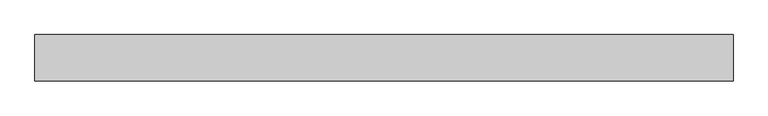
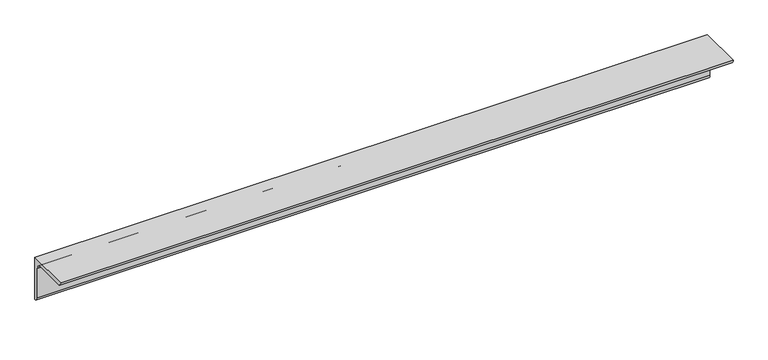
"""IFC4 building model written with IfcOpenShell, lengths in millimetres: member geometry, 0912_Steel Framing_L-KSD3502 : H_SB_AR_S04_L-100x100x10_KBR2."""

from ifc_helpers import new_model, si_unit, point, frame, frame_2d, origin, place, context, project, spatial, polyline, circle_curve, trimmed, segment, composite_curve, outline, extrude, source, transform, mapped, element, save


def member_c56ac2bd(model_context):
    return source(origin(), model_context, "Body", "SweptSolid", [
        extrude(outline(composite_curve([segment(polyline([(28.2, 28.2), (28.2, -71.8)]), True, "CONTINUOUS"), segment(trimmed(circle_curve(frame_2d((28.2, -61.8)), 10.0), [point((28.2, -71.8))], [point((18.2, -61.8))], False, "CARTESIAN"), True, "CONTINUOUS"), segment(polyline([(18.2, -61.8), (18.2, 8.2)]), True, "CONTINUOUS"), segment(trimmed(circle_curve(frame_2d((8.2, 8.2)), 10.0), [point((18.2, 8.2))], [point((8.2, 18.2))], True, "CARTESIAN"), True, "CONTINUOUS"), segment(polyline([(8.2, 18.2), (-61.8, 18.2)]), True, "CONTINUOUS"), segment(trimmed(circle_curve(frame_2d((-61.8, 28.2)), 10.0), [point((-61.8, 18.2))], [point((-71.8, 28.2))], False, "CARTESIAN"), True, "CONTINUOUS"), segment(polyline([(-71.8, 28.2), (28.2, 28.2)]), True, "CONTINUOUS")], self_intersect=False)), frame((-835.5368795, 0.0, 0.0), z_axis=(1.0, 0.0, 0.0), x_axis=(0.0, 1.0, 0.0)), (0.0, 0.0, 1.0), 1509.087639),
    ])


if __name__ == "__main__":
    model = new_model("IFC4")
    model_context = context("Model", 3, world=origin())
    ifc_project = project(units=[si_unit("LENGTHUNIT", "METRE", prefix="MILLI")], contexts=[model_context])
    site = spatial("IfcSite", under=ifc_project)
    building = spatial("IfcBuilding", under=site)
    placement = place(None, origin())
    member_shape = member_c56ac2bd(model_context)
    element("IfcMember", 1, ObjectType="0912_Steel Framing_L-KSD3502 : H_SB_AR_S04_L-100x100x10_KBR2", at=placement, inside=building, context=model_context, shape_type="MappedRepresentation", body=[
        mapped(member_shape, transform((0.0, 0.0, 0.0), x_axis=(1.0, 0.0, 0.0), y_axis=(0.0, 1.0, 0.0), z_axis=(0.0, 0.0, 1.0))),
    ])
    save(model, "model.ifc")

# Revit data of these elements
# Type "0912_Steel Framing_L-KSD3502 : H_SB_AR_S04_L-100x100x10_KBR2"
#   k = 25 mm
#   Perimeter = 0.40 m²/m
#   Nominal Weight = 14.90 kgf/m
#   Length [instance default] = 1000 mm
#   b = 100 mm
#   d = 100 mm
#   t = 10 mm
#   x = 28.2 mm
#   y = 28.2 mm
#   A = 1900.00 m²
#   Structural Material [instance default] = Steel, 45-345
# Element 1 (IfcMember, "0912_Steel Framing_L-KSD3502 : H_SB_AR_S04_L-100x100x10_KBR2")
#   Materials on its faces: "Steel, 45-345"
# Materials
#   "Steel, 45-345": class "Metal", colour RGB 189 187 185, transparency 0, Description = "Steel 345 MPa", Cost = 0
